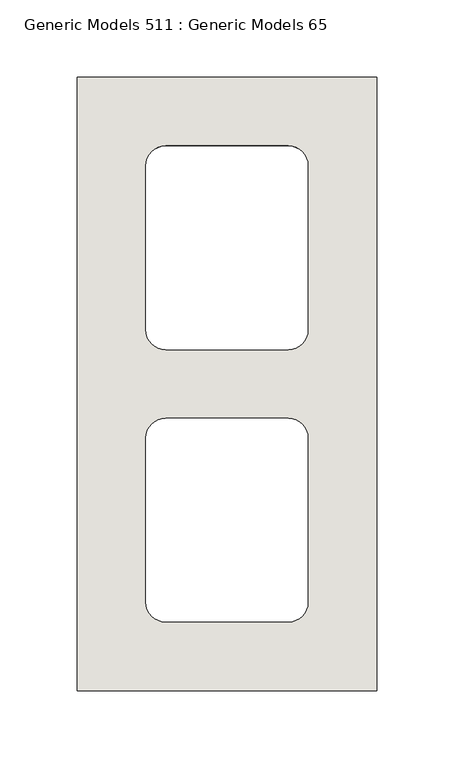
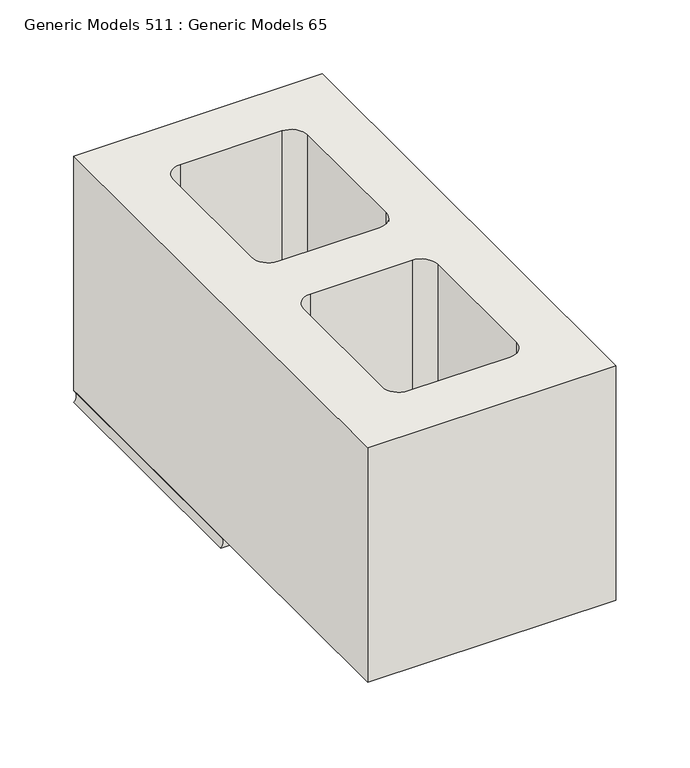
"""IFC4 building model written with IfcOpenShell, lengths in millimetres: wall geometry, Generic Models 511 : Generic Models 65."""

from ifc_helpers import new_model, si_unit, point, frame, frame_2d, origin, place, context, project, spatial, polyline, circle_curve, trimmed, segment, composite_curve, outline, extrude, source, transform, mapped, element, save
from ifc_brep_helpers import plane_surface, revolved_surface, advanced_brep


def generic_models_511_generic_models_65_1c3f84ec(model_context):
    return source(origin(), model_context, "Body", "SolidModel", [
        advanced_brep(
        [(428979.0125, 503.2375, 1635.125), (428785.3375, 503.2375, 1635.125), (428785.3375, 503.2375, 1625.6), (428979.0125, 503.2375, 1625.6), (428979.0125, 701.675, 1635.125), (428979.0125, 701.675, 1625.6), (428785.3375, 701.675, 1625.6), (428785.3375, 701.675, 1635.125), (428934.5625, 538.1625, 1635.125), (428921.8625, 525.4625, 1635.125), (428842.4875, 525.4625, 1635.125), (428829.7875, 538.1625, 1635.125), (428829.7875, 644.525, 1635.125), (428842.4875, 657.225, 1635.125), (428921.8625, 657.225, 1635.125), (428934.5625, 644.525, 1635.125), (428921.8625, 525.4625, 1625.6), (428934.5625, 538.1625, 1625.6), (428842.4875, 525.4625, 1625.6), (428829.7875, 538.1625, 1625.6), (428829.7875, 644.525, 1625.6), (428842.4875, 657.225, 1625.6), (428921.8625, 657.225, 1625.6), (428934.5625, 644.525, 1625.6)],
        [
            (0, 1),
            (1, 2, circle_curve(frame((428780.4545028, 503.2375, 1630.3625), z_axis=(0.0, 1.0, 0.0), x_axis=(1.0, 0.0, 0.0)), 6.8209287)),
            (2, 3),
            (3, 0, circle_curve(frame((428983.8954972, 503.2375, 1630.3625), z_axis=(0.0, 1.0, 0.0), x_axis=(-1.0, 0.0, 0.0)), 6.8209287)),
            (4, 5, circle_curve(frame((428983.8954972, 701.675, 1630.3625), z_axis=(0.0, -1.0, 0.0), x_axis=(-1.0, 0.0, 0.0)), 6.8209287)),
            (5, 6),
            (6, 7, circle_curve(frame((428780.4545028, 701.675, 1630.3625), z_axis=(0.0, -1.0, 0.0), x_axis=(1.0, 0.0, 0.0)), 6.8209287)),
            (7, 4),
            (0, 4),
            (7, 1),
            (8, 9, circle_curve(frame((428921.8625, 538.1625, 1635.125), z_axis=(0.0, 0.0, -1.0), x_axis=(-1.0, 0.0, 0.0)), 12.7)),
            (9, 10),
            (10, 11, circle_curve(frame((428842.4875, 538.1625, 1635.125), z_axis=(0.0, 0.0, -1.0), x_axis=(-1.0, 0.0, 0.0)), 12.7)),
            (11, 12),
            (12, 13, circle_curve(frame((428842.4875, 644.525, 1635.125), z_axis=(0.0, 0.0, -1.0), x_axis=(-1.0, 0.0, 0.0)), 12.7)),
            (13, 14),
            (14, 15, circle_curve(frame((428921.8625, 644.525, 1635.125), z_axis=(0.0, 0.0, -1.0), x_axis=(-1.0, 0.0, 0.0)), 12.7)),
            (15, 8),
            (16, 9),
            (8, 17),
            (17, 16, circle_curve(frame((428921.8625, 538.1625, 1625.6), z_axis=(0.0, 0.0, -1.0), x_axis=(-1.0, 0.0, 0.0)), 12.7)),
            (16, 18),
            (18, 10),
            (18, 19, circle_curve(frame((428842.4875, 538.1625, 1625.6), z_axis=(0.0, 0.0, -1.0), x_axis=(-1.0, 0.0, 0.0)), 12.7)),
            (19, 11),
            (19, 20),
            (20, 12),
            (20, 21, circle_curve(frame((428842.4875, 644.525, 1625.6), z_axis=(0.0, 0.0, -1.0), x_axis=(-1.0, 0.0, 0.0)), 12.7)),
            (21, 13),
            (21, 22),
            (22, 14),
            (22, 23, circle_curve(frame((428921.8625, 644.525, 1625.6), z_axis=(0.0, 0.0, -1.0), x_axis=(-1.0, 0.0, 0.0)), 12.7)),
            (23, 15),
            (23, 17),
            (6, 2),
            (5, 3),
        ],
        [
            plane_surface(frame((428882.175, 503.2375, 1635.521875), z_axis=(0.0, -1.0, 0.0), x_axis=(0.0, 0.0, 1.0))),
            plane_surface(frame((428882.175, 701.675, 1635.521875), z_axis=(0.0, 1.0, 0.0), x_axis=(0.0, 0.0, 1.0))),
            plane_surface(frame((428979.0125, 503.2375, 1635.125), z_axis=(0.0, 0.0, 1.0), x_axis=(0.0, 1.0, 0.0))),
            revolved_surface(polyline([(428909.1625, 538.1625, 1635.125), (428909.1625, 538.1625, 1625.6)]), (428921.8625, 538.1625, 1819.275), (0.0, 0.0, 1.0)),
            plane_surface(frame((428842.4875, 525.4625, 1819.275), z_axis=(0.0, 1.0, 0.0), x_axis=(0.0, 0.0, -1.0))),
            revolved_surface(polyline([(428829.7875, 538.1625, 1635.125), (428829.7875, 538.1625, 1625.6)]), (428842.4875, 538.1625, 1819.275), (0.0, 0.0, 1.0)),
            plane_surface(frame((428829.7875, 644.525, 1819.275), z_axis=(1.0, 0.0, 0.0), x_axis=(0.0, 0.0, -1.0))),
            revolved_surface(polyline([(428829.7875, 644.525, 1635.125), (428829.7875, 644.525, 1625.6)]), (428842.4875, 644.525, 1819.275), (0.0, 0.0, 1.0)),
            plane_surface(frame((428921.8625, 657.225, 1819.275), z_axis=(0.0, -1.0, 0.0), x_axis=(0.0, 0.0, -1.0))),
            revolved_surface(polyline([(428909.1625, 644.525, 1635.125), (428909.1625, 644.525, 1625.6)]), (428921.8625, 644.525, 1819.275), (0.0, 0.0, 1.0)),
            plane_surface(frame((428934.5625, 538.1625, 1819.275), z_axis=(-1.0, 0.0, 0.0), x_axis=(0.0, 0.0, -1.0))),
            revolved_surface(polyline([(428787.2754315, 701.675, 1630.3625), (428787.2754315, 503.2375, 1630.3625)]), (428780.4545028, 503.2375, 1630.3625), (0.0, 1.0, 0.0)),
            plane_surface(frame((428785.3375, 503.2375, 1625.6), z_axis=(0.0, 0.0, -1.0), x_axis=(0.0, 1.0, 0.0))),
            revolved_surface(polyline([(428977.07456850004, 701.675, 1630.3625), (428977.07456850004, 503.2375, 1630.3625)]), (428983.8954972, 503.2375, 1630.3625), (0.0, 1.0, 0.0)),
        ],
        [
            (0, [[1, 2, 3, 4]]),
            (1, [[5, 6, 7, 8]]),
            (2, [[-1, 9, -8, 10], [11, 12, 13, 14, 15, 16, 17, 18]]),
            (3, [[19, -11, 20, 21]]),
            (4, [[-19, 22, 23, -12]]),
            (5, [[-23, 24, 25, -13]]),
            (6, [[-25, 26, 27, -14]]),
            (7, [[-27, 28, 29, -15]]),
            (8, [[-29, 30, 31, -16]]),
            (9, [[-31, 32, 33, -17]]),
            (10, [[-33, 34, -20, -18]]),
            (11, [[-2, -10, -7, 35]]),
            (12, [[-3, -35, -6, 36], [-21, -34, -32, -30, -28, -26, -24, -22]]),
            (13, [[-4, -36, -5, -9]]),
        ],
    ),
        extrude(outline(polyline([(428979.0125, 304.8), (428785.3375, 304.8), (428785.3375, 701.675), (428979.0125, 701.675), (428979.0125, 304.8)]), holes=[composite_curve([segment(polyline([(428934.5625, 538.1625), (428934.5625, 644.525)]), True, "CONTINUOUS"), segment(trimmed(circle_curve(frame_2d((428921.8625, 644.525)), 12.7), [point((428934.5625, 644.525))], [point((428921.8625, 657.225))], True, "CARTESIAN"), True, "CONTINUOUS"), segment(polyline([(428921.8625, 657.225), (428842.4875, 657.225)]), True, "CONTINUOUS"), segment(trimmed(circle_curve(frame_2d((428842.4875, 644.525)), 12.7), [point((428842.4875, 657.225))], [point((428829.7875, 644.525))], True, "CARTESIAN"), True, "CONTINUOUS"), segment(polyline([(428829.7875, 644.525), (428829.7875, 538.1625)]), True, "CONTINUOUS"), segment(trimmed(circle_curve(frame_2d((428842.4875, 538.1625)), 12.7), [point((428829.7875, 538.1625))], [point((428842.4875, 525.4625))], True, "CARTESIAN"), True, "CONTINUOUS"), segment(polyline([(428842.4875, 525.4625), (428921.8625, 525.4625)]), True, "CONTINUOUS"), segment(trimmed(circle_curve(frame_2d((428921.8625, 538.1625)), 12.7), [point((428921.8625, 525.4625))], [point((428934.5625, 538.1625))], True, "CARTESIAN"), True, "CONTINUOUS")], self_intersect=False), composite_curve([segment(polyline([(428829.7875, 468.3125), (428829.7875, 361.95)]), True, "CONTINUOUS"), segment(trimmed(circle_curve(frame_2d((428842.4875, 361.95)), 12.7), [point((428829.7875, 361.95))], [point((428842.4875, 349.25))], True, "CARTESIAN"), True, "CONTINUOUS"), segment(polyline([(428842.4875, 349.25), (428921.8625, 349.25)]), True, "CONTINUOUS"), segment(trimmed(circle_curve(frame_2d((428921.8625, 361.95)), 12.7), [point((428921.8625, 349.25))], [point((428934.5625, 361.95))], True, "CARTESIAN"), True, "CONTINUOUS"), segment(polyline([(428934.5625, 361.95), (428934.5625, 468.3125)]), True, "CONTINUOUS"), segment(trimmed(circle_curve(frame_2d((428921.8625, 468.3125)), 12.7), [point((428934.5625, 468.3125))], [point((428921.8625, 481.0125))], True, "CARTESIAN"), True, "CONTINUOUS"), segment(polyline([(428921.8625, 481.0125), (428842.4875, 481.0125)]), True, "CONTINUOUS"), segment(trimmed(circle_curve(frame_2d((428842.4875, 468.3125)), 12.7), [point((428842.4875, 481.0125))], [point((428829.7875, 468.3125))], True, "CARTESIAN"), True, "CONTINUOUS")], self_intersect=False)]), frame((0.0, 0.0, 1635.125), z_axis=(0.0, 0.0, 1.0), x_axis=(1.0, 0.0, 0.0)), (0.0, 0.0, 1.0), 193.675),
    ])


if __name__ == "__main__":
    model = new_model("IFC4")
    model_context = context("Model", 3, world=origin())
    ifc_project = project(units=[si_unit("LENGTHUNIT", "METRE", prefix="MILLI")], contexts=[model_context])
    site = spatial("IfcSite", under=ifc_project)
    building = spatial("IfcBuilding", under=site)
    placement = place(None, origin())
    generic_models_511_generic_models_65_shape = generic_models_511_generic_models_65_1c3f84ec(model_context)
    element("IfcWall", 1, ObjectType="Generic Models 511 : Generic Models 65", at=placement, inside=building, context=model_context, shape_type="MappedRepresentation", body=[
        mapped(generic_models_511_generic_models_65_shape, transform((0.0, 0.0, 0.0), x_axis=(1.0, 0.0, 0.0), y_axis=(0.0, 1.0, 0.0), z_axis=(0.0, 0.0, 1.0))),
    ])
    save(model, "model.ifc")

# Revit data of these elements
# Element 1 (IfcWall, "Generic Models 511 : Generic Models 65")
#   Materials on its faces: "CMU (SEE 'WALL TAG' FOR SIZE)", "MORTAR JOINT"
# Materials
#   "CMU (SEE 'WALL TAG' FOR SIZE)": class "Masonry", colour RGB 203 203 199, transparency 0, Description = "Concrete masonry units", Cost = 0
#   "MORTAR JOINT": class "Generic", colour RGB 120 120 120, transparency 0, Cost = 0
